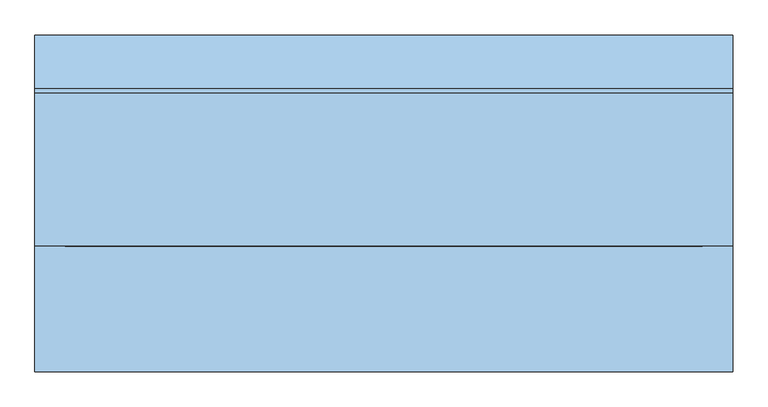
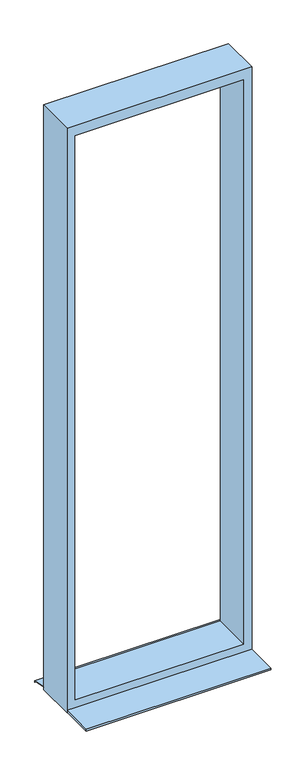
"""IFC4 building model written with IfcOpenShell, lengths in millimetres: window geometry, Fenster - Festverglasung : Feste Verglasung 4.58 x 1.37."""

from ifc_helpers import new_model, si_unit, frame, origin, place, context, project, spatial, polyline, outline, extrude, source, transform, mapped, element, save


def window_9186d0af(model_context):
    return source(origin(), model_context, "Body", "SweptSolid", [
        extrude(outline(polyline([(5580.0, 685.0), (5580.0, -685.0), (1000.0, -685.0), (1000.0, 685.0), (5580.0, 685.0)]), holes=[polyline([(5500.0, 625.0), (1080.0, 625.0), (1080.0, -625.0), (5500.0, -625.0), (5500.0, 625.0)])]), frame((0.0, -84.1317884, 0.0), z_axis=(0.0, 1.0, 0.0), x_axis=(0.0, 0.0, 1.0)), (0.0, 0.0, 1.0), 300.0),
        extrude(outline(polyline([(-685.0, -330.0), (-685.0, -84.1317884), (685.0, -84.1317884), (685.0, -330.0), (-685.0, -330.0)])), frame((0.0, 0.0, 1005.0), z_axis=(0.0, 0.0, 1.0), x_axis=(1.0, 0.0, 0.0)), (0.0, 0.0, 1.0), 15.0),
        extrude(outline(polyline([(225.8903659, 1020.0), (330.0, 1000.0), (330.0, 990.0), (328.0, 990.0), (328.0, 998.3604634), (225.6922839, 1018.0), (215.8682116, 1018.0), (215.8682116, 1020.0), (225.8903659, 1020.0)])), frame((-685.0, 0.0, 0.0), z_axis=(1.0, 0.0, 0.0), x_axis=(0.0, 1.0, 0.0)), (0.0, 0.0, 1.0), 1370.0),
    ])


if __name__ == "__main__":
    model = new_model("IFC4")
    model_context = context("Model", 3, world=origin())
    ifc_project = project(units=[si_unit("LENGTHUNIT", "METRE", prefix="MILLI")], contexts=[model_context])
    site = spatial("IfcSite", under=ifc_project)
    building = spatial("IfcBuilding", under=site)
    placement = place(None, origin())
    window_shape = window_9186d0af(model_context)
    element("IfcWindow", 1, ObjectType="Fenster - Festverglasung : Feste Verglasung 4.58 x 1.37", at=placement, inside=building, context=model_context, shape_type="MappedRepresentation", body=[
        mapped(window_shape, transform((0.0, 0.0, 0.0), x_axis=(1.0, 0.0, 0.0), y_axis=(0.0, 1.0, 0.0), z_axis=(0.0, 0.0, 1.0))),
    ])
    save(model, "model.ifc")

# Revit data of these elements
# Type "Fenster - Festverglasung : Feste Verglasung 4.58 x 1.37"
#   Type Mark = "59"
#   Operation = "SinglePanel"
#   Keynote = "16.05.01"
#   Visual Light Transmittance = 0.9
#   Solar Heat Gain Coefficient = 0.78
#   Rough Width = 1.370 m
#   Rough Height = 4.580 m
#   Heat Transfer Coefficient (U) = 3.6886 W/(m²·K)
#   Rahmentiefe = 0.300 m
#   Rahmenhöhe unten = 0.080 m
#   Höhe oberer  Rahmen = 0.080 m
#   Rahmenbreite = 0.060 m
#   Height = 4.580 m
#   Einbautiefe (von außen) [instance default] = 0.080 m
#   Width = 1.370 m
#   Wall Closure = 3
#   Bild [instance default] = none
#   Glas [instance default] = none
#   Innere Fensterbank [instance default] = none
#   Äußere Fensterbank [instance default] = none
#   Construction Type Id = ""
#   Analytic Construction = (empty or 0)
# Element 1 (IfcWindow, "Fenster - Festverglasung : Feste Verglasung 4.58 x 1.37")
#   Einbautiefe (von außen) = 0.084132 m
#   Materials on its faces: "Kunststoff - Weiß", "Holz - Birke"
# Materials
#   "Kunststoff - Weiß": class "Kunststoff", colour RGB 249 249 249, transparency 0, Cost = 0
#   "Holz - Birke": class "Holz", colour RGB 213 164 103, transparency 0, Cost = 0
